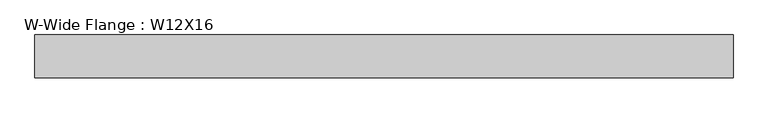
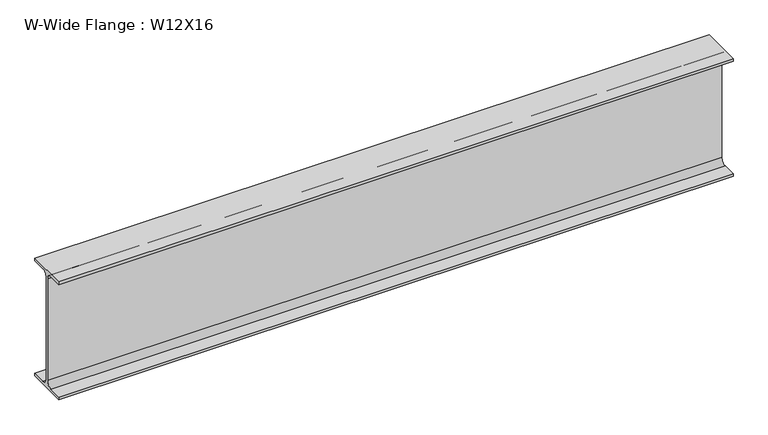
"""IFC4 building model written with IfcOpenShell, lengths in millimetres: beam geometry, W-Wide Flange : W12X16."""

from ifc_helpers import new_model, si_unit, point, frame, frame_2d, origin, place, context, project, spatial, polyline, circle_curve, trimmed, segment, composite_curve, outline, extrude, source, transform, mapped, element, save


def w_wide_flange_w12x16_f4fd3b0f(model_context):
    return source(origin(), model_context, "Body", "SweptSolid", [
        extrude(outline(composite_curve([segment(polyline([(50.673, -145.669), (50.673, -152.4), (-50.673, -152.4), (-50.673, -145.669), (-16.7005, -145.669)]), True, "CONTINUOUS"), segment(trimmed(circle_curve(frame_2d((-16.7005, -131.7625)), 13.9065), [point((-16.7005, -145.669))], [point((-2.794, -131.7625))], True, "CARTESIAN"), True, "CONTINUOUS"), segment(polyline([(-2.794, -131.7625), (-2.794, 131.7625)]), True, "CONTINUOUS"), segment(trimmed(circle_curve(frame_2d((-16.7005, 131.7625)), 13.9065), [point((-2.794, 131.7625))], [point((-16.7005, 145.669))], True, "CARTESIAN"), True, "CONTINUOUS"), segment(polyline([(-16.7005, 145.669), (-50.673, 145.669), (-50.673, 152.4), (50.673, 152.4), (50.673, 145.669), (16.7005, 145.669)]), True, "CONTINUOUS"), segment(trimmed(circle_curve(frame_2d((16.7005, 131.7625)), 13.9065), [point((16.7005, 145.669))], [point((2.794, 131.7625))], True, "CARTESIAN"), True, "CONTINUOUS"), segment(polyline([(2.794, 131.7625), (2.794, -131.7625)]), True, "CONTINUOUS"), segment(trimmed(circle_curve(frame_2d((16.7005, -131.7625)), 13.9065), [point((2.794, -131.7625))], [point((16.7005, -145.669))], True, "CARTESIAN"), True, "CONTINUOUS"), segment(polyline([(16.7005, -145.669), (50.673, -145.669)]), True, "CONTINUOUS")], self_intersect=False)), frame((-825.5, 0.0, 0.0), z_axis=(1.0, 0.0, 0.0), x_axis=(0.0, 1.0, 0.0)), (0.0, 0.0, 1.0), 1651.0),
    ])


if __name__ == "__main__":
    model = new_model("IFC4")
    model_context = context("Model", 3, world=origin())
    ifc_project = project(units=[si_unit("LENGTHUNIT", "METRE", prefix="MILLI")], contexts=[model_context])
    site = spatial("IfcSite", under=ifc_project)
    building = spatial("IfcBuilding", under=site)
    placement = place(None, origin())
    w_wide_flange_w12x16_shape = w_wide_flange_w12x16_f4fd3b0f(model_context)
    element("IfcBeam", 1, ObjectType="W-Wide Flange : W12X16", at=placement, inside=building, context=model_context, shape_type="MappedRepresentation", body=[
        mapped(w_wide_flange_w12x16_shape, transform((0.0, 0.0, 0.0), x_axis=(1.0, 0.0, 0.0), y_axis=(0.0, 1.0, 0.0), z_axis=(0.0, 0.0, 1.0))),
    ])
    save(model, "model.ifc")

# Revit data of these elements
# Type "W-Wide Flange : W12X16"
#   Assembly Code = "B10"
#   W = 16
#   Length [instance default] = 5' - 0"
#   bf = 0' - 3.99"
#   d = 1' - 0"
#   k = 0' - 0 13/16"
#   k2 = 0' - 0.5475"
#   tf = 0' - 0.265"
#   tw = 0' - 0.22"
#   A = 0.0327083 SF
#   Structural Material [instance default] = Steel ASTM A992
# Element 1 (IfcBeam, "W-Wide Flange : W12X16")
#   Materials on its faces: "Steel ASTM A992"
# Materials
#   "Steel ASTM A992": class "Metal", colour RGB 199 199 199, transparency 0, Description = "Structural steel 50ksi", Cost = 0
